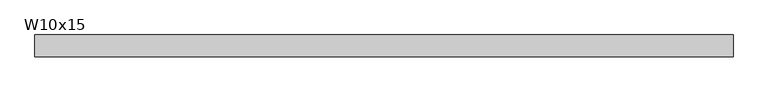
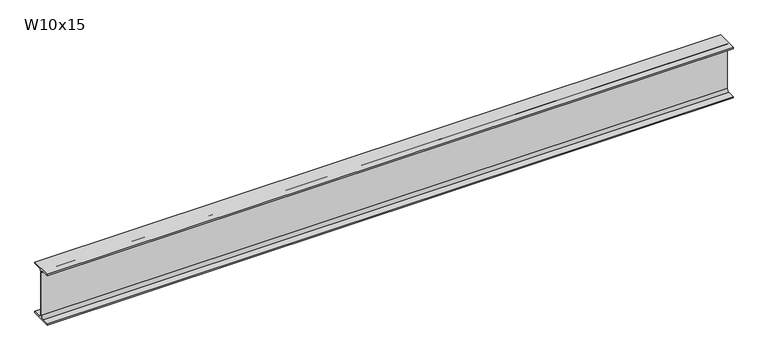
"""IFC4 building model written with IfcOpenShell, lengths in millimetres: beam geometry, RME W-Wide Flange : W10x15."""

from ifc_helpers import new_model, si_unit, point, frame, frame_2d, origin, place, context, project, spatial, polyline, circle_curve, trimmed, segment, composite_curve, outline, extrude, source, transform, mapped, element, save


def w10x15_c87059f4(model_context):
    return source(origin(), model_context, "Body", "SweptSolid", [
        extrude(outline(composite_curve([segment(polyline([(50.8, -120.142), (50.8, -127.0), (-50.8, -127.0), (-50.8, -120.142), (-16.7005, -120.142)]), True, "CONTINUOUS"), segment(trimmed(circle_curve(frame_2d((-16.7005, -106.3625)), 13.7795), [point((-16.7005, -120.142))], [point((-2.921, -106.3625))], True, "CARTESIAN"), True, "CONTINUOUS"), segment(polyline([(-2.921, -106.3625), (-2.921, 106.3625)]), True, "CONTINUOUS"), segment(trimmed(circle_curve(frame_2d((-16.7005, 106.3625)), 13.7795), [point((-2.921, 106.3625))], [point((-16.7005, 120.142))], True, "CARTESIAN"), True, "CONTINUOUS"), segment(polyline([(-16.7005, 120.142), (-50.8, 120.142), (-50.8, 127.0), (50.8, 127.0), (50.8, 120.142), (16.7005, 120.142)]), True, "CONTINUOUS"), segment(trimmed(circle_curve(frame_2d((16.7005, 106.3625)), 13.7795), [point((16.7005, 120.142))], [point((2.921, 106.3625))], True, "CARTESIAN"), True, "CONTINUOUS"), segment(polyline([(2.921, 106.3625), (2.921, -106.3625)]), True, "CONTINUOUS"), segment(trimmed(circle_curve(frame_2d((16.7005, -106.3625)), 13.7795), [point((2.921, -106.3625))], [point((16.7005, -120.142))], True, "CARTESIAN"), True, "CONTINUOUS"), segment(polyline([(16.7005, -120.142), (50.8, -120.142)]), True, "CONTINUOUS")], self_intersect=False)), frame((-1577.9778256, 0.0, 0.0), z_axis=(1.0, 0.0, 0.0), x_axis=(0.0, 1.0, 0.0)), (0.0, 0.0, 1.0), 3246.5960434),
    ])


if __name__ == "__main__":
    model = new_model("IFC4")
    model_context = context("Model", 3, world=origin())
    ifc_project = project(units=[si_unit("LENGTHUNIT", "METRE", prefix="MILLI")], contexts=[model_context])
    site = spatial("IfcSite", under=ifc_project)
    building = spatial("IfcBuilding", under=site)
    placement = place(None, origin())
    w10x15_shape = w10x15_c87059f4(model_context)
    element("IfcBeam", 1, ObjectType="RME W-Wide Flange : W10x15", at=placement, inside=building, context=model_context, shape_type="MappedRepresentation", body=[
        mapped(w10x15_shape, transform((0.0, 0.0, 0.0), x_axis=(1.0, 0.0, 0.0), y_axis=(0.0, 1.0, 0.0), z_axis=(0.0, 0.0, 1.0))),
    ])
    save(model, "model.ifc")

# Revit data of these elements
# Type "RME W-Wide Flange : W10x15"
#   WELD P [instance default] = ""
#   WELD LE [instance default] = ""
#   WELD D [instance default] = ""
#   TOP SECTION SIZE [instance default] = ""
#   TOP SECTION LENGTH [instance default] = ""
#   REMARKS [instance default] = ""
#   REINF TYPE [instance default] = ""
#   Nominal Size = "W24"
#   End Bearing Capacity [instance default] = ""
#   BOT SECTION SIZE [instance default] = ""
#   BOT SECTION LENGTH [instance default] = ""
#   Assembly Code = "B10"
#   W = 15
#   Start Extension Calculation [instance default] = 10' - 0"
#   Start Extension [instance default] = -0' - 0 1/2"
#   End Extension Calculation [instance default] = 10' - 0"
#   End Extension [instance default] = -0' - 0 1/2"
#   Length [instance default] = 5' - 0"
#   bf = 0' - 4"
#   d = 0' - 10"
#   k = 0' - 0 13/16"
#   k2 = 0' - 0.5425"
#   tf = 0' - 0.27"
#   tw = 0' - 0.23"
#   A = 0.030625 SF
#   Structural Material [instance default] = Metal - Steel - ASTM A992
# Element 1 (IfcBeam, "RME W-Wide Flange : W10x15")
#   Start Extension Calculation = 9' - 8.43148"
#   Start Extension = -0' - 4.06852"
#   Length = 10' - 11.38726"
#   Materials on its faces: "Metal - Steel - ASTM A992"
# Materials
#   "Metal - Steel - ASTM A992": class "Metal", colour RGB 255 128 0, transparency 0
